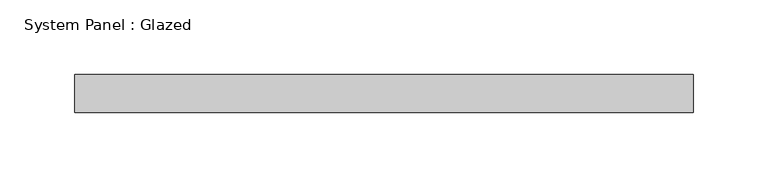
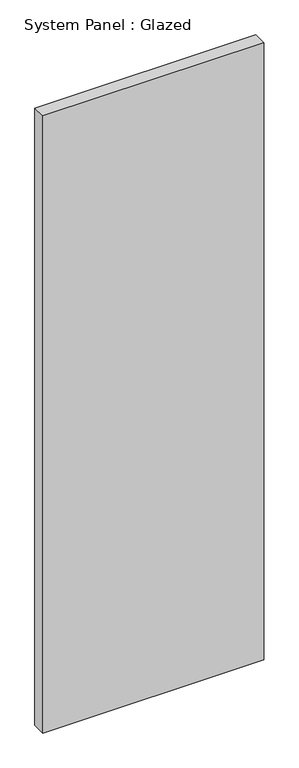
"""IFC4 building model written with IfcOpenShell, lengths in millimetres: plate geometry, System Panel : Glazed."""

from ifc_helpers import new_model, si_unit, origin, origin_with_axes, place, context, project, spatial, polyline, outline, extrude, source, transform, mapped, element, save


def system_panel_glazed_be080e7e(model_context):
    return source(origin(), model_context, "Body", "SweptSolid", [
        extrude(outline(polyline([(206.3749998, 19.05), (-206.3749998, 19.05), (-206.3749998, 44.45), (206.3749998, 44.45), (206.3749998, 19.05)])), origin_with_axes(), (0.0, 0.0, 1.0), 1219.2),
    ])


if __name__ == "__main__":
    model = new_model("IFC4")
    model_context = context("Model", 3, world=origin())
    ifc_project = project(units=[si_unit("LENGTHUNIT", "METRE", prefix="MILLI")], contexts=[model_context])
    site = spatial("IfcSite", under=ifc_project)
    building = spatial("IfcBuilding", under=site)
    placement = place(None, origin())
    system_panel_glazed_shape = system_panel_glazed_be080e7e(model_context)
    element("IfcPlate", 1, ObjectType="System Panel : Glazed", at=placement, inside=building, context=model_context, shape_type="MappedRepresentation", body=[
        mapped(system_panel_glazed_shape, transform((0.0, 0.0, 0.0), x_axis=(1.0, 0.0, 0.0), y_axis=(0.0, 1.0, 0.0), z_axis=(0.0, 0.0, 1.0))),
    ])
    save(model, "model.ifc")

# Revit data of these elements
# Element 1 (IfcPlate, "System Panel : Glazed")
#   Materials on its faces: "Glass"
# Materials
#   "Glass": class "Glass", colour RGB 0 128 192, transparency 0.75
